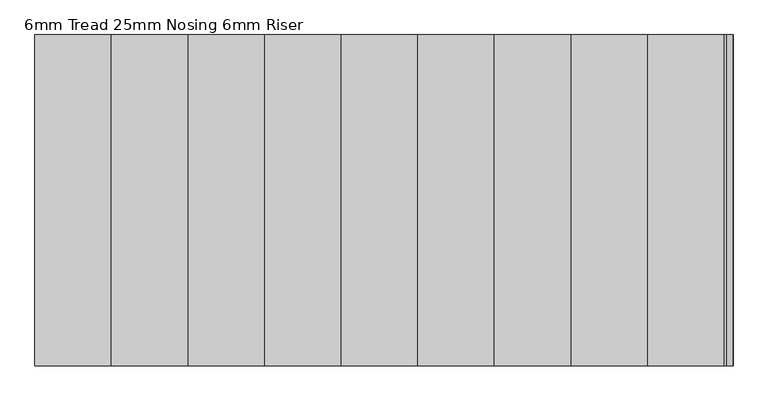
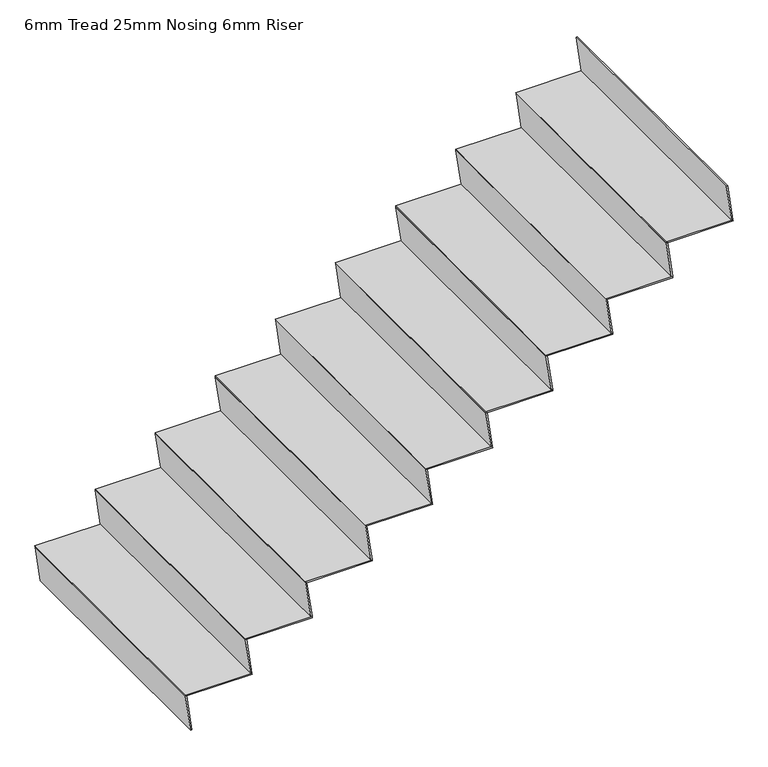
"""IFC4 building model written with IfcOpenShell, lengths in millimetres: stair flight geometry, 6mm Tread 25mm Nosing 6mm Riser."""

import ifcopenshell
import ifcopenshell.guid

model = None  # the IFC model being written
_history = None  # IfcOwnerHistory: only IFC2X3 demands one
_inside = {}  # id of a spatial element -> (the spatial element, [elements in it])
_under = {}  # id of a project, library or spatial element -> (it, [spatial elements below it])
_declared = {}  # id of a project -> (the project, [libraries it declares])
_typed = {}  # id of a type object -> (the type object, [elements of that type])
_made_of = {}  # id of a material, layer set ... -> (it, [elements and type objects made of it])


def new_model(schema):
    """Start an empty IFC model of exactly this schema.

    Asked for "IFC4X3", IfcOpenShell would pick the latest addendum, in which some entities
    have other attributes; the version numbers below select the first issue.
    IFC2X3 requires an IfcOwnerHistory on every rooted entity: one is made here for all.
    """
    global model, _history
    if schema == "IFC4X3":
        model = ifcopenshell.file(schema_version=(4, 3, 0, 0))
    else:
        model = ifcopenshell.file(schema=schema)
    _inside.clear()
    _under.clear()
    _declared.clear()
    _typed.clear()
    _made_of.clear()
    _history = None
    if model.schema == "IFC2X3":
        org = make("IfcOrganization", Name="unknown")
        user = make(
            "IfcPersonAndOrganization",
            ThePerson=make("IfcPerson", FamilyName="unknown"),
            TheOrganization=org,
        )
        app = make(
            "IfcApplication",
            ApplicationDeveloper=org,
            Version="unknown",
            ApplicationFullName="unknown",
            ApplicationIdentifier="unknown",
        )
        _history = make(
            "IfcOwnerHistory",
            OwningUser=user,
            OwningApplication=app,
            ChangeAction="ADDED",
            CreationDate=0,
        )
    return model


def make(cls, **values):
    """One entity of the class cls with the attributes given. An attribute that is None is left unset."""
    return model.create_entity(
        cls, **{name: value for name, value in values.items() if value is not None}
    )


def rooted(cls, **values):
    """An entity with a GlobalId (a new one), such as an element, a storey or a relation."""
    return make(cls, GlobalId=ifcopenshell.guid.new(), OwnerHistory=_history, **values)


def si_unit(unit_type, name, prefix=None):
    """IfcSIUnit, for example si_unit("LENGTHUNIT", "METRE", prefix="MILLI")."""
    return make("IfcSIUnit", UnitType=unit_type, Prefix=prefix, Name=name)


def assignment(units):
    """IfcUnitAssignment: the units of a project."""
    return None if units is None else make("IfcUnitAssignment", Units=units)


def point(xyz):
    """IfcCartesianPoint."""
    return None if xyz is None else make("IfcCartesianPoint", Coordinates=xyz)


def direction(xyz):
    """IfcDirection."""
    return None if xyz is None else make("IfcDirection", DirectionRatios=xyz)


def frame(location, z_axis=None, x_axis=None):
    """IfcAxis2Placement3D, a coordinate frame: its origin and axes. An axis left out is left unset."""
    return make(
        "IfcAxis2Placement3D",
        Location=point(location),
        Axis=direction(z_axis),
        RefDirection=direction(x_axis),
    )


def origin():
    """The frame at (0, 0, 0) with its axes left unset."""
    return frame((0.0, 0.0, 0.0))


def place(relative_to, where):
    """IfcLocalPlacement: puts the frame where relative to a parent placement (None: the world)."""
    return make(
        "IfcLocalPlacement", PlacementRelTo=relative_to, RelativePlacement=where
    )


def context(
    kind, dimensions, precision=None, world=None, true_north=None, identifier=None
):
    """IfcGeometricRepresentationContext, for example the 3D "Model" context."""
    return make(
        "IfcGeometricRepresentationContext",
        ContextIdentifier=identifier,
        ContextType=kind,
        CoordinateSpaceDimension=dimensions,
        Precision=precision,
        WorldCoordinateSystem=world,
        TrueNorth=true_north,
    )


def project(units=None, contexts=None):
    """IfcProject with its units and contexts."""
    return rooted(
        "IfcProject",
        Name="project",
        RepresentationContexts=contexts,
        UnitsInContext=assignment(units),
    )


def spatial(cls, under=None, at=None, **own):
    """A site, building, storey or space (cls), placed at a placement, below another one or the project."""
    s = rooted(cls, ObjectPlacement=at, **own)
    if under is not None:
        _under.setdefault(under.id(), (under, []))[1].append(s)
    return s


def polyline(points):
    """IfcPolyline through the points."""
    return make("IfcPolyline", Points=[point(p) for p in points])


def outline(outer, holes=None, kind="AREA"):
    """IfcArbitraryClosedProfileDef: a profile drawn as a closed curve; with holes, ...WithVoids."""
    if holes is None:
        return make("IfcArbitraryClosedProfileDef", ProfileType=kind, OuterCurve=outer)
    return make(
        "IfcArbitraryProfileDefWithVoids",
        ProfileType=kind,
        OuterCurve=outer,
        InnerCurves=holes,
    )


def extrude(swept, where, along, depth):
    """IfcExtrudedAreaSolid: the profile swept, set in the frame where, extruded along a direction by depth."""
    return make(
        "IfcExtrudedAreaSolid",
        SweptArea=swept,
        Position=where,
        ExtrudedDirection=direction(along),
        Depth=depth,
    )


def shape(context_of_items, identifier, shape_type, items):
    """IfcShapeRepresentation: the items that make up one representation, for example the "Body"."""
    return make(
        "IfcShapeRepresentation",
        ContextOfItems=context_of_items,
        RepresentationIdentifier=identifier,
        RepresentationType=shape_type,
        Items=items,
    )


def source(mapping_origin, context_of_items, identifier, shape_type, items):
    """IfcRepresentationMap: a shape defined once, which mapped items show again and again."""
    return make(
        "IfcRepresentationMap",
        MappingOrigin=mapping_origin,
        MappedRepresentation=shape(context_of_items, identifier, shape_type, items),
    )


def transform(
    local_origin,
    x_axis=None,
    y_axis=None,
    z_axis=None,
    scale=None,
    scale2=None,
    scale3=None,
    uniform=True,
):
    """IfcCartesianTransformationOperator3D, or its non-uniform kind. x_axis, y_axis, z_axis: its Axis1, 2, 3."""
    if uniform:
        return make(
            "IfcCartesianTransformationOperator3D",
            Axis1=direction(x_axis),
            Axis2=direction(y_axis),
            LocalOrigin=point(local_origin),
            Scale=scale,
            Axis3=direction(z_axis),
        )
    return make(
        "IfcCartesianTransformationOperator3DnonUniform",
        Axis1=direction(x_axis),
        Axis2=direction(y_axis),
        LocalOrigin=point(local_origin),
        Scale=scale,
        Axis3=direction(z_axis),
        Scale2=scale2,
        Scale3=scale3,
    )


def mapped(mapping_source, mapping_target):
    """IfcMappedItem: shows the shape of a source again, moved by a transform."""
    return make(
        "IfcMappedItem", MappingSource=mapping_source, MappingTarget=mapping_target
    )


def made_of(thing, what):
    """Note that an element or type object is made of a material, layer set ...; save() writes the relation."""
    if what is not None:
        _made_of.setdefault(what.id(), (what, []))[1].append(thing)
    return thing


def element(
    cls,
    number,
    at=None,
    inside=None,
    cuts=None,
    type_object=None,
    material=None,
    context=None,
    identifier="Body",
    shape_type=None,
    held_by="IfcProductDefinitionShape",
    body=None,
    shapes=None,
    **own,
):
    """One element of the class cls, such as IfcWall. Its Tag is "e" and its number.

    at: its placement. inside: the storey or other place that contains it. cuts: it is an
    opening in that element (IfcRelVoidsElement). A single representation is given by context,
    identifier, shape_type and body (its items); several are given by shapes. held_by: the class
    of the entity that holds the representations. save() writes the other relations.
    """
    e = rooted(cls, Tag="e%d" % number, ObjectPlacement=at, **own)
    if body is not None:
        shapes = [shape(context, identifier, shape_type, body)]
    if shapes is not None:
        e.Representation = make(held_by, Representations=shapes)
    if inside is not None:
        _inside.setdefault(inside.id(), (inside, []))[1].append(e)
    if cuts is not None:
        rooted(
            "IfcRelVoidsElement", RelatingBuildingElement=cuts, RelatedOpeningElement=e
        )
    if type_object is not None:
        _typed.setdefault(type_object.id(), (type_object, []))[1].append(e)
    return made_of(e, material)


def aggregate(whole, parts):
    """IfcRelAggregates: a whole, such as a stair, and the parts it consists of."""
    return rooted("IfcRelAggregates", RelatingObject=whole, RelatedObjects=parts)


def save(model, path):
    """Write the relations noted so far, then the file.

    IfcRelAggregates (storeys below a building ...), IfcRelContainedInSpatialStructure (elements
    in a storey), IfcRelDefinesByType, IfcRelAssociatesMaterial and IfcRelDeclares: one each for
    every whole, place, type object, material and project.
    """
    for whole, parts in _under.values():
        aggregate(whole, parts)
    for where, things in _inside.values():
        rooted(
            "IfcRelContainedInSpatialStructure",
            RelatedElements=things,
            RelatingStructure=where,
        )
    for kind, things in _typed.values():
        rooted("IfcRelDefinesByType", RelatedObjects=things, RelatingType=kind)
    for what, things in _made_of.values():
        rooted("IfcRelAssociatesMaterial", RelatedObjects=things, RelatingMaterial=what)
    for by, libraries in _declared.values():
        rooted("IfcRelDeclares", RelatingContext=by, RelatedDefinitions=libraries)
    model.write(path)


def stair_flight_6mm_tread_25mm_nosing_6mm_riser_dd128cf0(model_context):
    return source(origin(), model_context, "Body", "SweptSolid", [
        extrude(outline(polyline([(6400.0, -16043.9409643), (6400.0, -16350.0), (6394.0, -16349.15625), (6394.0, -16043.0972143), (6400.0, -16043.9409643)])), frame((0.0, 12030.4345331, 0.0), z_axis=(0.0, 1.0, 0.0), x_axis=(0.0, 0.0, 1.0)), (0.0, 0.0, 1.0), 1190.0),
        extrude(outline(polyline([(6394.0, -16349.15625), (6222.2222222, -16325.0), (6222.2222222, -16318.9409643), (6394.0, -16343.0972143), (6394.0, -16349.15625)])), frame((0.0, 12030.4345331, 0.0), z_axis=(0.0, 1.0, 0.0), x_axis=(0.0, 0.0, 1.0)), (0.0, 0.0, 1.0), 1190.0),
        extrude(outline(polyline([(6571.7777778, -16074.15625), (6400.0, -16050.0), (6400.0, -16043.9409643), (6571.7777778, -16068.0972143), (6571.7777778, -16074.15625)])), frame((0.0, 12030.4345331, 0.0), z_axis=(0.0, 1.0, 0.0), x_axis=(0.0, 0.0, 1.0)), (0.0, 0.0, 1.0), 1190.0),
        extrude(outline(polyline([(6577.7777778, -15768.9409643), (6577.7777778, -16075.0), (6571.7777778, -16074.15625), (6571.7777778, -15768.0972143), (6577.7777778, -15768.9409643)])), frame((0.0, 12030.4345331, 0.0), z_axis=(0.0, 1.0, 0.0), x_axis=(0.0, 0.0, 1.0)), (0.0, 0.0, 1.0), 1190.0),
        extrude(outline(polyline([(6749.5555556, -15799.15625), (6577.7777778, -15775.0), (6577.7777778, -15768.9409643), (6749.5555556, -15793.0972143), (6749.5555556, -15799.15625)])), frame((0.0, 12030.4345331, 0.0), z_axis=(0.0, 1.0, 0.0), x_axis=(0.0, 0.0, 1.0)), (0.0, 0.0, 1.0), 1190.0),
        extrude(outline(polyline([(6755.5555556, -15493.9409643), (6755.5555556, -15800.0), (6749.5555556, -15799.15625), (6749.5555556, -15493.0972143), (6755.5555556, -15493.9409643)])), frame((0.0, 12030.4345331, 0.0), z_axis=(0.0, 1.0, 0.0), x_axis=(0.0, 0.0, 1.0)), (0.0, 0.0, 1.0), 1190.0),
        extrude(outline(polyline([(6927.3333333, -15524.15625), (6755.5555556, -15500.0), (6755.5555556, -15493.9409643), (6927.3333333, -15518.0972143), (6927.3333333, -15524.15625)])), frame((0.0, 12030.4345331, 0.0), z_axis=(0.0, 1.0, 0.0), x_axis=(0.0, 0.0, 1.0)), (0.0, 0.0, 1.0), 1190.0),
        extrude(outline(polyline([(6933.3333333, -15218.9409643), (6933.3333333, -15525.0), (6927.3333333, -15524.15625), (6927.3333333, -15218.0972143), (6933.3333333, -15218.9409643)])), frame((0.0, 12030.4345331, 0.0), z_axis=(0.0, 1.0, 0.0), x_axis=(0.0, 0.0, 1.0)), (0.0, 0.0, 1.0), 1190.0),
        extrude(outline(polyline([(7105.1111111, -15249.15625), (6933.3333333, -15225.0), (6933.3333333, -15218.9409643), (7105.1111111, -15243.0972143), (7105.1111111, -15249.15625)])), frame((0.0, 12030.4345331, 0.0), z_axis=(0.0, 1.0, 0.0), x_axis=(0.0, 0.0, 1.0)), (0.0, 0.0, 1.0), 1190.0),
        extrude(outline(polyline([(7111.1111111, -14943.9409643), (7111.1111111, -15250.0), (7105.1111111, -15249.15625), (7105.1111111, -14943.0972143), (7111.1111111, -14943.9409643)])), frame((0.0, 12030.4345331, 0.0), z_axis=(0.0, 1.0, 0.0), x_axis=(0.0, 0.0, 1.0)), (0.0, 0.0, 1.0), 1190.0),
        extrude(outline(polyline([(7282.8888889, -14974.15625), (7111.1111111, -14950.0), (7111.1111111, -14943.9409643), (7282.8888889, -14968.0972143), (7282.8888889, -14974.15625)])), frame((0.0, 12030.4345331, 0.0), z_axis=(0.0, 1.0, 0.0), x_axis=(0.0, 0.0, 1.0)), (0.0, 0.0, 1.0), 1190.0),
        extrude(outline(polyline([(7288.8888889, -14668.9409643), (7288.8888889, -14975.0), (7282.8888889, -14974.15625), (7282.8888889, -14668.0972143), (7288.8888889, -14668.9409643)])), frame((0.0, 12030.4345331, 0.0), z_axis=(0.0, 1.0, 0.0), x_axis=(0.0, 0.0, 1.0)), (0.0, 0.0, 1.0), 1190.0),
        extrude(outline(polyline([(7460.6666667, -14699.15625), (7288.8888889, -14675.0), (7288.8888889, -14668.9409643), (7460.6666667, -14693.0972143), (7460.6666667, -14699.15625)])), frame((0.0, 12030.4345331, 0.0), z_axis=(0.0, 1.0, 0.0), x_axis=(0.0, 0.0, 1.0)), (0.0, 0.0, 1.0), 1190.0),
        extrude(outline(polyline([(7466.6666667, -14393.9409643), (7466.6666667, -14700.0), (7460.6666667, -14699.15625), (7460.6666667, -14393.0972143), (7466.6666667, -14393.9409643)])), frame((0.0, 12030.4345331, 0.0), z_axis=(0.0, 1.0, 0.0), x_axis=(0.0, 0.0, 1.0)), (0.0, 0.0, 1.0), 1190.0),
        extrude(outline(polyline([(7638.4444444, -14424.15625), (7466.6666667, -14400.0), (7466.6666667, -14393.9409643), (7638.4444444, -14418.0972143), (7638.4444444, -14424.15625)])), frame((0.0, 12030.4345331, 0.0), z_axis=(0.0, 1.0, 0.0), x_axis=(0.0, 0.0, 1.0)), (0.0, 0.0, 1.0), 1190.0),
        extrude(outline(polyline([(7644.4444444, -14118.9409643), (7644.4444444, -14425.0), (7638.4444444, -14424.15625), (7638.4444444, -14118.0972143), (7644.4444444, -14118.9409643)])), frame((0.0, 12030.4345331, 0.0), z_axis=(0.0, 1.0, 0.0), x_axis=(0.0, 0.0, 1.0)), (0.0, 0.0, 1.0), 1190.0),
        extrude(outline(polyline([(7816.2222222, -14149.15625), (7644.4444444, -14125.0), (7644.4444444, -14118.9409643), (7816.2222222, -14143.0972143), (7816.2222222, -14149.15625)])), frame((0.0, 12030.4345331, 0.0), z_axis=(0.0, 1.0, 0.0), x_axis=(0.0, 0.0, 1.0)), (0.0, 0.0, 1.0), 1190.0),
        extrude(outline(polyline([(7994.0, -13874.15625), (7822.2222222, -13850.0), (7822.2222222, -13843.9409643), (7994.0, -13868.0972143), (7994.0, -13874.15625)])), frame((0.0, 12030.4345331, 0.0), z_axis=(0.0, 1.0, 0.0), x_axis=(0.0, 0.0, 1.0)), (0.0, 0.0, 1.0), 1190.0),
        extrude(outline(polyline([(7822.2222222, -13843.9409643), (7822.2222222, -14150.0), (7816.2222222, -14149.15625), (7816.2222222, -13843.0972143), (7822.2222222, -13843.9409643)])), frame((0.0, 12030.4345331, 0.0), z_axis=(0.0, 1.0, 0.0), x_axis=(0.0, 0.0, 1.0)), (0.0, 0.0, 1.0), 1190.0),
    ])


if __name__ == "__main__":
    model = new_model("IFC4")
    model_context = context("Model", 3, world=origin())
    ifc_project = project(units=[si_unit("LENGTHUNIT", "METRE", prefix="MILLI")], contexts=[model_context])
    site = spatial("IfcSite", under=ifc_project)
    building = spatial("IfcBuilding", under=site)
    placement = place(None, origin())
    stair_flight_6mm_tread_25mm_nosing_6mm_riser_shape = stair_flight_6mm_tread_25mm_nosing_6mm_riser_dd128cf0(model_context)
    element("IfcStairFlight", 1, ObjectType="6mm Tread 25mm Nosing 6mm Riser", at=placement, inside=building, context=model_context, shape_type="MappedRepresentation", body=[
        mapped(stair_flight_6mm_tread_25mm_nosing_6mm_riser_shape, transform((0.0, 0.0, 0.0), x_axis=(1.0, 0.0, 0.0), y_axis=(0.0, 1.0, 0.0), z_axis=(0.0, 0.0, 1.0))),
    ])
    save(model, "model.ifc")

# Revit data of these elements
# Element 1 (IfcStairFlight, "6mm Tread 25mm Nosing 6mm Riser")
#   Materials on its faces: "Steel, Paint Finish, Dark Gray"
# Materials
#   "Steel, Paint Finish, Dark Gray": class "Metal", colour RGB 89 89 89, transparency 0, Description = "Steel, paint finish, dark gray, glossy", Cost = 0
